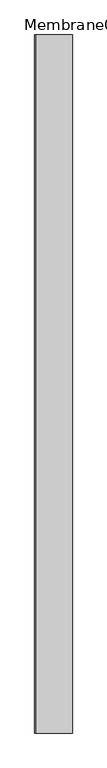
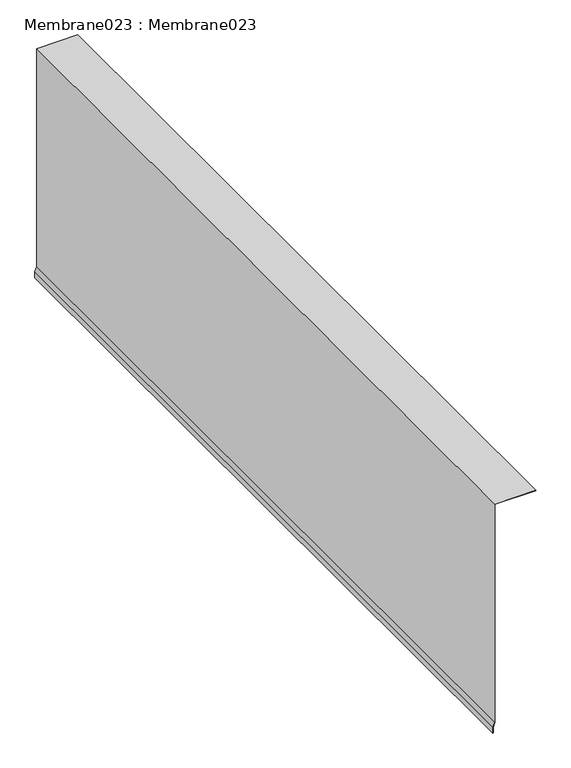
"""IFC4 building model written with IfcOpenShell, lengths in millimetres: proxy geometry, Membrane023 : Membrane023."""

from ifc_helpers import new_model, si_unit, frame, origin, place, context, project, spatial, polyline, outline, extrude, source, transform, mapped, element, save


def membrane023_membrane023_29a42501(model_context):
    return source(origin(), model_context, "Body", "SweptSolid", [
        extrude(outline(polyline([(40160.8681333, -7122.8238703), (40160.8681333, -7226.5656531), (39579.4993977, -7226.5656531), (39568.2741325, -7230.6513155), (39552.6918208, -7230.6513155), (39552.6918208, -7229.6513155), (39568.0978055, -7229.6513155), (39579.3230707, -7225.5656531), (40159.8681333, -7225.5656531), (40159.8681333, -7122.8238703), (40160.8681333, -7122.8238703)])), frame((0.0, 7982.1531721, 0.0), z_axis=(0.0, 1.0, 0.0), x_axis=(0.0, 0.0, 1.0)), (0.0, 0.0, 1.0), 2000.0),
    ])


if __name__ == "__main__":
    model = new_model("IFC4")
    model_context = context("Model", 3, world=origin())
    ifc_project = project(units=[si_unit("LENGTHUNIT", "METRE", prefix="MILLI")], contexts=[model_context])
    site = spatial("IfcSite", under=ifc_project)
    building = spatial("IfcBuilding", under=site)
    placement = place(None, origin())
    membrane023_membrane023_shape = membrane023_membrane023_29a42501(model_context)
    element("IfcBuildingElementProxy", 1, Name="Membrane023 : Membrane023", ObjectType="Membrane023 : Membrane023", at=placement, inside=building, context=model_context, shape_type="MappedRepresentation", body=[
        mapped(membrane023_membrane023_shape, transform((0.0, 0.0, 0.0), x_axis=(1.0, 0.0, 0.0), y_axis=(0.0, 1.0, 0.0), z_axis=(0.0, 0.0, 1.0))),
    ])
    save(model, "model.ifc")

# Revit data of these elements
# Type "Membrane023 : Membrane023"
#   NameOverride = "Membrane023"
# Element 1 (IfcBuildingElementProxy, "Membrane023 : Membrane023")
#   Materials on its faces: "2 LAYERS NO. 30 ASTM D226 ASPHALT SATURATED ORGANIC FELT"
# Materials
#   "2 LAYERS NO. 30 ASTM D226 ASPHALT SATURATED ORGANIC FELT": class "Unassigned", colour RGB 46 171 0, transparency 0
